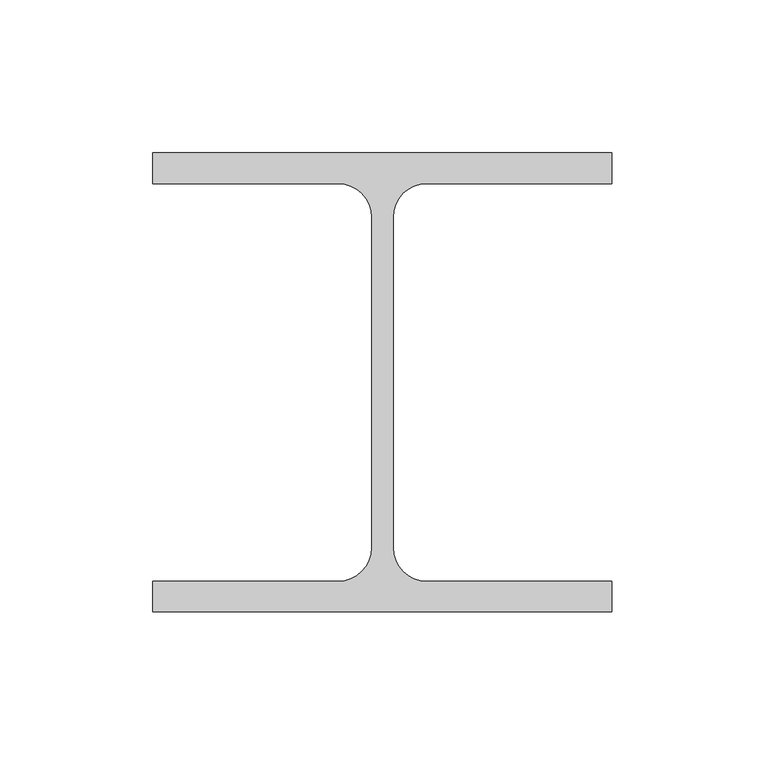
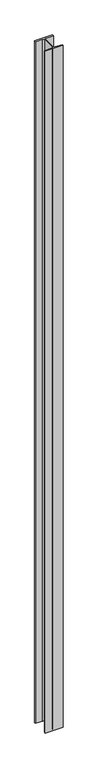
"""IFC4 building model written with IfcOpenShell, lengths in millimetres: column geometry, Steel Column_H_KSD3502 : H_SC_ASC_H-150x150x7x10."""

import ifcopenshell
import ifcopenshell.guid

model = None  # the IFC model being written
_history = None  # IfcOwnerHistory: only IFC2X3 demands one
_inside = {}  # id of a spatial element -> (the spatial element, [elements in it])
_under = {}  # id of a project, library or spatial element -> (it, [spatial elements below it])
_declared = {}  # id of a project -> (the project, [libraries it declares])
_typed = {}  # id of a type object -> (the type object, [elements of that type])
_made_of = {}  # id of a material, layer set ... -> (it, [elements and type objects made of it])


def new_model(schema):
    """Start an empty IFC model of exactly this schema.

    Asked for "IFC4X3", IfcOpenShell would pick the latest addendum, in which some entities
    have other attributes; the version numbers below select the first issue.
    IFC2X3 requires an IfcOwnerHistory on every rooted entity: one is made here for all.
    """
    global model, _history
    if schema == "IFC4X3":
        model = ifcopenshell.file(schema_version=(4, 3, 0, 0))
    else:
        model = ifcopenshell.file(schema=schema)
    _inside.clear()
    _under.clear()
    _declared.clear()
    _typed.clear()
    _made_of.clear()
    _history = None
    if model.schema == "IFC2X3":
        org = make("IfcOrganization", Name="unknown")
        user = make(
            "IfcPersonAndOrganization",
            ThePerson=make("IfcPerson", FamilyName="unknown"),
            TheOrganization=org,
        )
        app = make(
            "IfcApplication",
            ApplicationDeveloper=org,
            Version="unknown",
            ApplicationFullName="unknown",
            ApplicationIdentifier="unknown",
        )
        _history = make(
            "IfcOwnerHistory",
            OwningUser=user,
            OwningApplication=app,
            ChangeAction="ADDED",
            CreationDate=0,
        )
    return model


def make(cls, **values):
    """One entity of the class cls with the attributes given. An attribute that is None is left unset."""
    return model.create_entity(
        cls, **{name: value for name, value in values.items() if value is not None}
    )


def rooted(cls, **values):
    """An entity with a GlobalId (a new one), such as an element, a storey or a relation."""
    return make(cls, GlobalId=ifcopenshell.guid.new(), OwnerHistory=_history, **values)


def si_unit(unit_type, name, prefix=None):
    """IfcSIUnit, for example si_unit("LENGTHUNIT", "METRE", prefix="MILLI")."""
    return make("IfcSIUnit", UnitType=unit_type, Prefix=prefix, Name=name)


def assignment(units):
    """IfcUnitAssignment: the units of a project."""
    return None if units is None else make("IfcUnitAssignment", Units=units)


def point(xyz):
    """IfcCartesianPoint."""
    return None if xyz is None else make("IfcCartesianPoint", Coordinates=xyz)


def direction(xyz):
    """IfcDirection."""
    return None if xyz is None else make("IfcDirection", DirectionRatios=xyz)


def frame(location, z_axis=None, x_axis=None):
    """IfcAxis2Placement3D, a coordinate frame: its origin and axes. An axis left out is left unset."""
    return make(
        "IfcAxis2Placement3D",
        Location=point(location),
        Axis=direction(z_axis),
        RefDirection=direction(x_axis),
    )


def frame_2d(location, x_axis=None):
    """IfcAxis2Placement2D, a coordinate frame in the plane: its origin and x axis."""
    return make(
        "IfcAxis2Placement2D", Location=point(location), RefDirection=direction(x_axis)
    )


def origin():
    """The frame at (0, 0, 0) with its axes left unset."""
    return frame((0.0, 0.0, 0.0))


def place(relative_to, where):
    """IfcLocalPlacement: puts the frame where relative to a parent placement (None: the world)."""
    return make(
        "IfcLocalPlacement", PlacementRelTo=relative_to, RelativePlacement=where
    )


def context(
    kind, dimensions, precision=None, world=None, true_north=None, identifier=None
):
    """IfcGeometricRepresentationContext, for example the 3D "Model" context."""
    return make(
        "IfcGeometricRepresentationContext",
        ContextIdentifier=identifier,
        ContextType=kind,
        CoordinateSpaceDimension=dimensions,
        Precision=precision,
        WorldCoordinateSystem=world,
        TrueNorth=true_north,
    )


def project(units=None, contexts=None):
    """IfcProject with its units and contexts."""
    return rooted(
        "IfcProject",
        Name="project",
        RepresentationContexts=contexts,
        UnitsInContext=assignment(units),
    )


def spatial(cls, under=None, at=None, **own):
    """A site, building, storey or space (cls), placed at a placement, below another one or the project."""
    s = rooted(cls, ObjectPlacement=at, **own)
    if under is not None:
        _under.setdefault(under.id(), (under, []))[1].append(s)
    return s


def polyline(points):
    """IfcPolyline through the points."""
    return make("IfcPolyline", Points=[point(p) for p in points])


def circle_curve(where, radius):
    """IfcCircle in the frame where."""
    return make("IfcCircle", Position=where, Radius=radius)


def trimmed(basis, trim1, trim2, sense, master):
    """IfcTrimmedCurve: the piece of a basis curve between two trims."""
    return make(
        "IfcTrimmedCurve",
        BasisCurve=basis,
        Trim1=trim1,
        Trim2=trim2,
        SenseAgreement=sense,
        MasterRepresentation=master,
    )


def segment(curve, same_sense, transition):
    """IfcCompositeCurveSegment."""
    return make(
        "IfcCompositeCurveSegment",
        Transition=transition,
        SameSense=same_sense,
        ParentCurve=curve,
    )


def composite_curve(segments, self_intersect=None):
    """IfcCompositeCurve: segments joined end to end."""
    return make("IfcCompositeCurve", Segments=segments, SelfIntersect=self_intersect)


def outline(outer, holes=None, kind="AREA"):
    """IfcArbitraryClosedProfileDef: a profile drawn as a closed curve; with holes, ...WithVoids."""
    if holes is None:
        return make("IfcArbitraryClosedProfileDef", ProfileType=kind, OuterCurve=outer)
    return make(
        "IfcArbitraryProfileDefWithVoids",
        ProfileType=kind,
        OuterCurve=outer,
        InnerCurves=holes,
    )


def extrude(swept, where, along, depth):
    """IfcExtrudedAreaSolid: the profile swept, set in the frame where, extruded along a direction by depth."""
    return make(
        "IfcExtrudedAreaSolid",
        SweptArea=swept,
        Position=where,
        ExtrudedDirection=direction(along),
        Depth=depth,
    )


def shape(context_of_items, identifier, shape_type, items):
    """IfcShapeRepresentation: the items that make up one representation, for example the "Body"."""
    return make(
        "IfcShapeRepresentation",
        ContextOfItems=context_of_items,
        RepresentationIdentifier=identifier,
        RepresentationType=shape_type,
        Items=items,
    )


def source(mapping_origin, context_of_items, identifier, shape_type, items):
    """IfcRepresentationMap: a shape defined once, which mapped items show again and again."""
    return make(
        "IfcRepresentationMap",
        MappingOrigin=mapping_origin,
        MappedRepresentation=shape(context_of_items, identifier, shape_type, items),
    )


def transform(
    local_origin,
    x_axis=None,
    y_axis=None,
    z_axis=None,
    scale=None,
    scale2=None,
    scale3=None,
    uniform=True,
):
    """IfcCartesianTransformationOperator3D, or its non-uniform kind. x_axis, y_axis, z_axis: its Axis1, 2, 3."""
    if uniform:
        return make(
            "IfcCartesianTransformationOperator3D",
            Axis1=direction(x_axis),
            Axis2=direction(y_axis),
            LocalOrigin=point(local_origin),
            Scale=scale,
            Axis3=direction(z_axis),
        )
    return make(
        "IfcCartesianTransformationOperator3DnonUniform",
        Axis1=direction(x_axis),
        Axis2=direction(y_axis),
        LocalOrigin=point(local_origin),
        Scale=scale,
        Axis3=direction(z_axis),
        Scale2=scale2,
        Scale3=scale3,
    )


def mapped(mapping_source, mapping_target):
    """IfcMappedItem: shows the shape of a source again, moved by a transform."""
    return make(
        "IfcMappedItem", MappingSource=mapping_source, MappingTarget=mapping_target
    )


def made_of(thing, what):
    """Note that an element or type object is made of a material, layer set ...; save() writes the relation."""
    if what is not None:
        _made_of.setdefault(what.id(), (what, []))[1].append(thing)
    return thing


def element(
    cls,
    number,
    at=None,
    inside=None,
    cuts=None,
    type_object=None,
    material=None,
    context=None,
    identifier="Body",
    shape_type=None,
    held_by="IfcProductDefinitionShape",
    body=None,
    shapes=None,
    **own,
):
    """One element of the class cls, such as IfcWall. Its Tag is "e" and its number.

    at: its placement. inside: the storey or other place that contains it. cuts: it is an
    opening in that element (IfcRelVoidsElement). A single representation is given by context,
    identifier, shape_type and body (its items); several are given by shapes. held_by: the class
    of the entity that holds the representations. save() writes the other relations.
    """
    e = rooted(cls, Tag="e%d" % number, ObjectPlacement=at, **own)
    if body is not None:
        shapes = [shape(context, identifier, shape_type, body)]
    if shapes is not None:
        e.Representation = make(held_by, Representations=shapes)
    if inside is not None:
        _inside.setdefault(inside.id(), (inside, []))[1].append(e)
    if cuts is not None:
        rooted(
            "IfcRelVoidsElement", RelatingBuildingElement=cuts, RelatedOpeningElement=e
        )
    if type_object is not None:
        _typed.setdefault(type_object.id(), (type_object, []))[1].append(e)
    return made_of(e, material)


def aggregate(whole, parts):
    """IfcRelAggregates: a whole, such as a stair, and the parts it consists of."""
    return rooted("IfcRelAggregates", RelatingObject=whole, RelatedObjects=parts)


def save(model, path):
    """Write the relations noted so far, then the file.

    IfcRelAggregates (storeys below a building ...), IfcRelContainedInSpatialStructure (elements
    in a storey), IfcRelDefinesByType, IfcRelAssociatesMaterial and IfcRelDeclares: one each for
    every whole, place, type object, material and project.
    """
    for whole, parts in _under.values():
        aggregate(whole, parts)
    for where, things in _inside.values():
        rooted(
            "IfcRelContainedInSpatialStructure",
            RelatedElements=things,
            RelatingStructure=where,
        )
    for kind, things in _typed.values():
        rooted("IfcRelDefinesByType", RelatedObjects=things, RelatingType=kind)
    for what, things in _made_of.values():
        rooted("IfcRelAssociatesMaterial", RelatedObjects=things, RelatingMaterial=what)
    for by, libraries in _declared.values():
        rooted("IfcRelDeclares", RelatingContext=by, RelatedDefinitions=libraries)
    model.write(path)


def column_5fc823e1(model_context):
    return source(origin(), model_context, "Body", "SweptSolid", [
        extrude(outline(composite_curve([segment(polyline([(75.0, 75.0), (75.0, 65.0), (14.5, 65.0)]), True, "CONTINUOUS"), segment(trimmed(circle_curve(frame_2d((14.5, 54.0)), 11.0), [point((14.5, 65.0))], [point((3.5, 54.0))], True, "CARTESIAN"), True, "CONTINUOUS"), segment(polyline([(3.5, 54.0), (3.5, -54.0)]), True, "CONTINUOUS"), segment(trimmed(circle_curve(frame_2d((14.5, -54.0)), 11.0), [point((3.5, -54.0))], [point((14.5, -65.0))], True, "CARTESIAN"), True, "CONTINUOUS"), segment(polyline([(14.5, -65.0), (75.0, -65.0), (75.0, -75.0), (-75.0, -75.0), (-75.0, -65.0), (-14.5, -65.0)]), True, "CONTINUOUS"), segment(trimmed(circle_curve(frame_2d((-14.5, -54.0)), 11.0), [point((-14.5, -65.0))], [point((-3.5, -54.0))], True, "CARTESIAN"), True, "CONTINUOUS"), segment(polyline([(-3.5, -54.0), (-3.5, 54.0)]), True, "CONTINUOUS"), segment(trimmed(circle_curve(frame_2d((-14.5, 54.0)), 11.0), [point((-3.5, 54.0))], [point((-14.5, 65.0))], True, "CARTESIAN"), True, "CONTINUOUS"), segment(polyline([(-14.5, 65.0), (-75.0, 65.0), (-75.0, 75.0), (75.0, 75.0)]), True, "CONTINUOUS")], self_intersect=False)), frame((0.0, 0.0, 599.9720055), z_axis=(0.0, 0.0, 1.0), x_axis=(1.0, 0.0, 0.0)), (0.0, 0.0, 1.0), 6000.0),
    ])


if __name__ == "__main__":
    model = new_model("IFC4")
    model_context = context("Model", 3, world=origin())
    ifc_project = project(units=[si_unit("LENGTHUNIT", "METRE", prefix="MILLI")], contexts=[model_context])
    site = spatial("IfcSite", under=ifc_project)
    building = spatial("IfcBuilding", under=site)
    placement = place(None, origin())
    column_shape = column_5fc823e1(model_context)
    element("IfcColumn", 1, ObjectType="Steel Column_H_KSD3502 : H_SC_ASC_H-150x150x7x10", at=placement, inside=building, context=model_context, shape_type="MappedRepresentation", body=[
        mapped(column_shape, transform((0.0, 0.0, 0.0), x_axis=(1.0, 0.0, 0.0), y_axis=(0.0, 1.0, 0.0), z_axis=(0.0, 0.0, 1.0))),
    ])
    save(model, "model.ifc")

# Revit data of these elements
# Type "Steel Column_H_KSD3502 : H_SC_ASC_H-150x150x7x10"
#   Width = 15.0 cm
#   Web Thickness = 0.7 cm
#   Web Fillet = 1.1 cm
#   Warping Constant = 27562.5 cm⁶
#   Torsional Moment of Inertia = 11.6007 cm⁴
#   Section Area = 40.14 cm²
#   Plastic Modulus weak axis = 115.0 cm³
#   Plastic Modulus strong axis = 246.0 cm³
#   Perimeter = 1.27 m²/m
#   Nominal Weight = 31.50 kgf/m
#   Moment of Inertia weak axis = 563.00 cm⁴
#   Moment of Inertia strong axis = 1640.00 cm⁴
#   Height = 15.0 cm
#   Flange Thickness = 1.0 cm
#   Elastic Modulus weak axis = 75.1 cm³
#   Elastic Modulus strong axis = 219.0 cm³
#   Centroid Vertical = 7.5 cm
#   Centroid Horizontal = 7.5 cm
#   Bolt Spacing = 13.97 cm
#   Structural Material [instance default] = Steel, 45-345
#   Section Name Key = ""
#   Assembly Code = ""
# Element 1 (IfcColumn, "Steel Column_H_KSD3502 : H_SC_ASC_H-150x150x7x10")
#   Structural Material = A03AD029-00005_Anchor Bolt (Installation only)_M24
#   Materials on its faces: "A03AD029-00005_Anchor Bolt (Installation only)_M24"
# Materials
#   "Steel, 45-345": class "Metal", colour RGB 189 187 185, transparency 0, Description = "Steel 345 MPa", Cost = 0
#   "A03AD029-00005_Anchor Bolt (Installation only)_M24": class "Unassigned", colour RGB 84 83 81, transparency 0, Cost = 0
